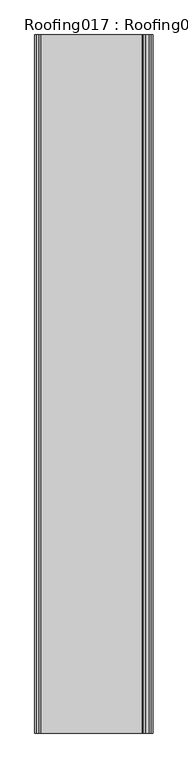
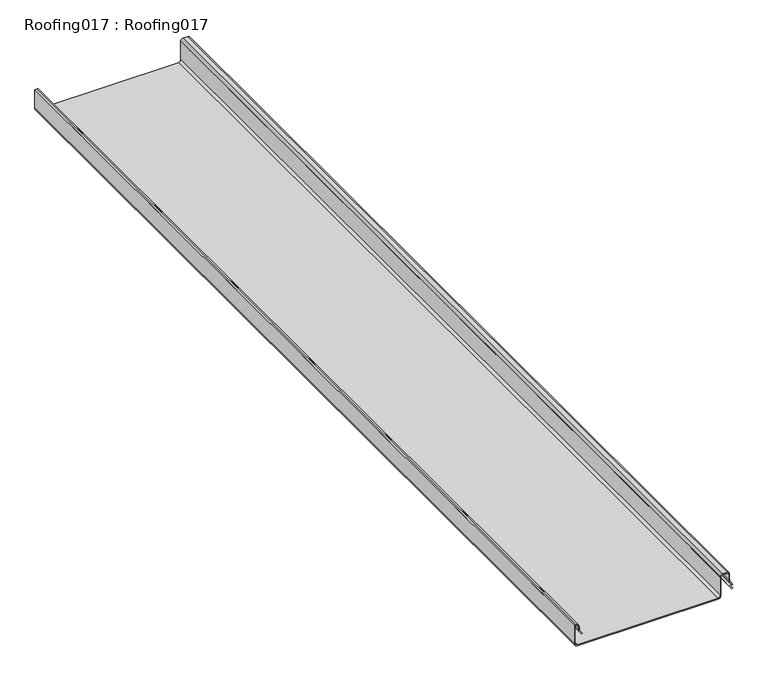
"""IFC4 building model written with IfcOpenShell, lengths in millimetres: proxy geometry, Roofing017 : Roofing017."""

from ifc_helpers import new_model, si_unit, point, frame, frame_2d, origin, place, context, project, spatial, polyline, circle_curve, trimmed, segment, composite_curve, outline, extrude, source, transform, mapped, element, save


def roofing017_roofing017_ac897961(model_context):
    return source(origin(), model_context, "Body", "SweptSolid", [
        extrude(outline(composite_curve([segment(polyline([(41810.80004, 5509.3259297), (41802.3258778, 5515.4735783), (41803.5002989, 5517.0924467), (41811.974461, 5510.9447981)]), True, "CONTINUOUS"), segment(trimmed(circle_curve(frame_2d((41813.7830695, 5513.4378556)), 3.08), [point((41811.974461, 5510.9447981))], [point((41813.7830695, 5510.3578556))], True, "CARTESIAN"), True, "CONTINUOUS"), segment(polyline([(41813.7830695, 5510.3578556), (41820.5396278, 5510.3578556)]), True, "CONTINUOUS"), segment(trimmed(circle_curve(frame_2d((41820.5396278, 5503.2778556)), 7.08), [point((41820.5396278, 5510.3578556))], [point((41827.6196278, 5503.2778556))], False, "CARTESIAN"), True, "CONTINUOUS"), segment(polyline([(41827.6196278, 5503.2778556), (41827.6196278, 5499.6830509), (41785.8824403, 5499.6830509)]), True, "CONTINUOUS"), segment(trimmed(circle_curve(frame_2d((41785.8824403, 5506.7630509)), 7.08), [point((41785.8824403, 5499.6830509))], [point((41778.8024403, 5506.7630509))], False, "CARTESIAN"), True, "CONTINUOUS"), segment(polyline([(41778.8024403, 5506.7630509), (41778.8024403, 5807.0371329)]), True, "CONTINUOUS"), segment(trimmed(circle_curve(frame_2d((41785.8824403, 5807.0371329)), 7.08), [point((41778.8024403, 5807.0371329))], [point((41785.8824403, 5814.1171329))], False, "CARTESIAN"), True, "CONTINUOUS"), segment(polyline([(41785.8824403, 5814.1171329), (41827.4958778, 5814.1171329)]), True, "CONTINUOUS"), segment(trimmed(circle_curve(frame_2d((41827.4958778, 5817.1971329)), 3.08), [point((41827.4958778, 5814.1171329))], [point((41830.5758778, 5817.1971329))], True, "CARTESIAN"), True, "CONTINUOUS"), segment(polyline([(41830.5758778, 5817.1971329), (41830.5758778, 5827.2049098)]), True, "CONTINUOUS"), segment(trimmed(circle_curve(frame_2d((41827.4958778, 5827.2049098)), 3.08), [point((41830.5758778, 5827.2049098))], [point((41827.4958778, 5830.2849098))], True, "CARTESIAN"), True, "CONTINUOUS"), segment(polyline([(41827.4958778, 5830.2849098), (41814.3133037, 5830.2849098)]), True, "CONTINUOUS"), segment(trimmed(circle_curve(frame_2d((41814.3133037, 5837.3649098)), 7.08), [point((41814.3133037, 5830.2849098))], [point((41810.8234609, 5831.2047639))], False, "CARTESIAN"), True, "CONTINUOUS"), segment(polyline([(41810.8234609, 5831.2047639), (41801.98033, 5836.21457), (41799.4289318, 5831.8629052), (41792.0466166, 5837.1332296), (41793.2086903, 5838.7609841), (41798.8102528, 5834.7619606), (41801.2516591, 5838.9260231), (41811.8092922, 5832.9449181)]), True, "CONTINUOUS"), segment(trimmed(circle_curve(frame_2d((41814.3133037, 5837.3649098)), 5.08), [point((41811.8092922, 5832.9449181))], [point((41814.3133037, 5832.2849098))], True, "CARTESIAN"), True, "CONTINUOUS"), segment(polyline([(41814.3133037, 5832.2849098), (41827.4958778, 5832.2849098)]), True, "CONTINUOUS"), segment(trimmed(circle_curve(frame_2d((41827.4958778, 5827.2049098)), 5.08), [point((41827.4958778, 5832.2849098))], [point((41832.5758778, 5827.2049098))], False, "CARTESIAN"), True, "CONTINUOUS"), segment(polyline([(41832.5758778, 5827.2049098), (41832.5758778, 5817.1971329)]), True, "CONTINUOUS"), segment(trimmed(circle_curve(frame_2d((41827.4958778, 5817.1971329)), 5.08), [point((41832.5758778, 5817.1971329))], [point((41827.4958778, 5812.1171329))], False, "CARTESIAN"), True, "CONTINUOUS"), segment(polyline([(41827.4958778, 5812.1171329), (41785.8824403, 5812.1171329)]), True, "CONTINUOUS"), segment(trimmed(circle_curve(frame_2d((41785.8824403, 5807.0371329)), 5.08), [point((41785.8824403, 5812.1171329))], [point((41780.8024403, 5807.0371329))], True, "CARTESIAN"), True, "CONTINUOUS"), segment(polyline([(41780.8024403, 5807.0371329), (41780.8024403, 5506.7630509)]), True, "CONTINUOUS"), segment(trimmed(circle_curve(frame_2d((41785.8824403, 5506.7630509)), 5.08), [point((41780.8024403, 5506.7630509))], [point((41785.8824403, 5501.6830509))], True, "CARTESIAN"), True, "CONTINUOUS"), segment(polyline([(41785.8824403, 5501.6830509), (41825.6196278, 5501.6830509), (41825.6196278, 5503.2778556)]), True, "CONTINUOUS"), segment(trimmed(circle_curve(frame_2d((41820.5396278, 5503.2778556)), 5.08), [point((41825.6196278, 5503.2778556))], [point((41820.5396278, 5508.3578556))], True, "CARTESIAN"), True, "CONTINUOUS"), segment(polyline([(41820.5396278, 5508.3578556), (41813.7830695, 5508.3578556)]), True, "CONTINUOUS"), segment(trimmed(circle_curve(frame_2d((41813.7830695, 5513.4378556)), 5.08), [point((41813.7830695, 5508.3578556))], [point((41810.80004, 5509.3259297))], False, "CARTESIAN"), True, "CONTINUOUS")], self_intersect=False)), frame((0.0, 2217.3609988, 0.0), z_axis=(0.0, 1.0, 0.0), x_axis=(0.0, 0.0, 1.0)), (0.0, 0.0, 1.0), 2000.0),
    ])


if __name__ == "__main__":
    model = new_model("IFC4")
    model_context = context("Model", 3, world=origin())
    ifc_project = project(units=[si_unit("LENGTHUNIT", "METRE", prefix="MILLI")], contexts=[model_context])
    site = spatial("IfcSite", under=ifc_project)
    building = spatial("IfcBuilding", under=site)
    placement = place(None, origin())
    roofing017_roofing017_shape = roofing017_roofing017_ac897961(model_context)
    element("IfcBuildingElementProxy", 1, Name="Roofing017 : Roofing017", ObjectType="Roofing017 : Roofing017", at=placement, inside=building, context=model_context, shape_type="MappedRepresentation", body=[
        mapped(roofing017_roofing017_shape, transform((0.0, 0.0, 0.0), x_axis=(1.0, 0.0, 0.0), y_axis=(0.0, 1.0, 0.0), z_axis=(0.0, 0.0, 1.0))),
    ])
    save(model, "model.ifc")

# Revit data of these elements
# Type "Roofing017 : Roofing017"
#   NameOverride = "Roofing017"
# Element 1 (IfcBuildingElementProxy, "Roofing017 : Roofing017")
#   Materials on its faces: "STANDING SEAM METAL ROOF FOLLOW MANU. RECOMMENDED EDGE/TRANSITION DETAILS"
# Materials
#   "STANDING SEAM METAL ROOF FOLLOW MANU. RECOMMENDED EDGE/TRANSITION DETAILS": class "Unassigned", colour RGB 128 128 128, transparency 0, Cost = 0
